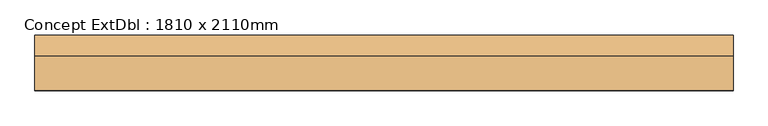
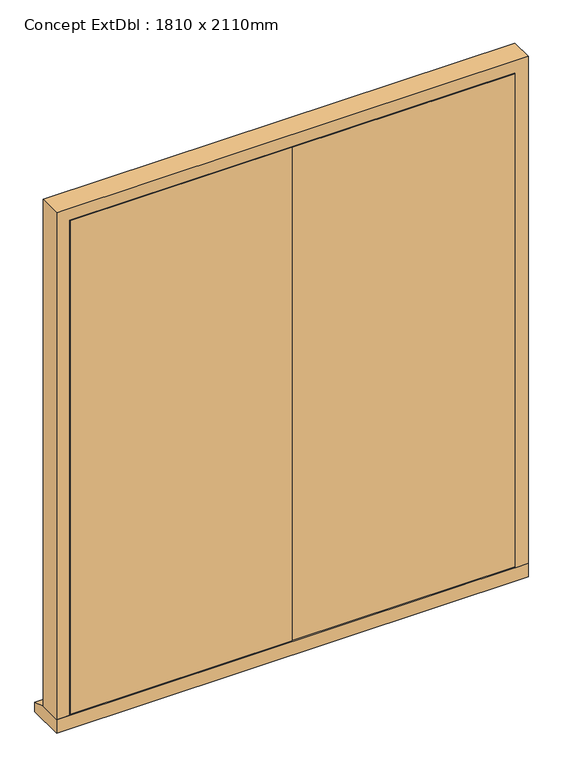
"""IFC4 building model written with IfcOpenShell, lengths in millimetres: door geometry, Concept ExtDbl : 1810 x 2110mm."""

from ifc_helpers import new_model, si_unit, frame, origin, place, context, project, spatial, polyline, outline, extrude, faceted_brep, source, transform, mapped, element, save


def concept_extdbl_1810_x_2110mm_abc10830(model_context):
    return source(origin(), model_context, "Body", "SolidModel", [
        faceted_brep([(834.5, 190.0, 54.5), (905.0, 190.0, 54.5), (905.0, 101.0, 54.5), (856.5, 101.0, 54.5), (856.5, 148.0, 54.5), (834.5, 148.0, 54.5), (834.5, 190.0, 2039.5), (-834.5, 190.0, 2039.5), (-834.5, 190.0, 54.5), (-905.0, 190.0, 54.5), (-905.0, 190.0, 2110.0), (905.0, 190.0, 2110.0), (905.0, 101.0, 2110.0), (-905.0, 101.0, 2110.0), (-905.0, 101.0, 54.5), (-856.5, 101.0, 54.5), (-856.5, 101.0, 2061.5), (856.5, 101.0, 2061.5), (856.5, 148.0, 2061.5), (-856.5, 148.0, 2061.5), (-856.5, 148.0, 54.5), (-834.5, 148.0, 54.5), (-834.5, 148.0, 2039.5), (834.5, 148.0, 2039.5)], [[[0, 1, 2, 3, 4, 5]], [[1, 0, 6, 7, 8, 9, 10, 11]], [[2, 1, 11, 12]], [[3, 2, 12, 13, 14, 15, 16, 17]], [[4, 3, 17, 18]], [[5, 4, 18, 19, 20, 21, 22, 23]], [[0, 5, 23, 6]], [[7, 22, 21, 8]], [[8, 21, 20, 15, 14, 9]], [[13, 10, 9, 14]], [[19, 16, 15, 20]], [[12, 11, 10, 13]], [[18, 17, 16, 19]], [[6, 23, 22, 7]]]),
        extrude(outline(polyline([(101.0, 0.0), (101.0, 54.5), (190.0, 54.5), (245.0, 38.5947221), (245.0, 0.0), (101.0, 0.0)])), frame((-905.0, 0.0, 0.0), z_axis=(1.0, 0.0, 0.0), x_axis=(0.0, 1.0, 0.0)), (0.0, 0.0, 1.0), 1810.0),
        extrude(outline(polyline([(853.5, 101.0), (1.5, 101.0), (1.5, 145.0), (853.5, 145.0), (853.5, 101.0)])), frame((0.0, 0.0, 58.5), z_axis=(0.0, 0.0, 1.0), x_axis=(1.0, 0.0, 0.0)), (0.0, 0.0, 1.0), 2000.0),
        extrude(outline(polyline([(-1.5, 101.0), (-853.5, 101.0), (-853.5, 145.0), (-1.5, 145.0), (-1.5, 101.0)])), frame((0.0, 0.0, 58.5), z_axis=(0.0, 0.0, 1.0), x_axis=(1.0, 0.0, 0.0)), (0.0, 0.0, 1.0), 2000.0),
    ])


if __name__ == "__main__":
    model = new_model("IFC4")
    model_context = context("Model", 3, world=origin())
    ifc_project = project(units=[si_unit("LENGTHUNIT", "METRE", prefix="MILLI")], contexts=[model_context])
    site = spatial("IfcSite", under=ifc_project)
    building = spatial("IfcBuilding", under=site)
    placement = place(None, origin())
    concept_extdbl_1810_x_2110mm_shape = concept_extdbl_1810_x_2110mm_abc10830(model_context)
    element("IfcDoor", 1, ObjectType="Concept ExtDbl : 1810 x 2110mm", at=placement, inside=building, context=model_context, shape_type="MappedRepresentation", body=[
        mapped(concept_extdbl_1810_x_2110mm_shape, transform((0.0, 0.0, 0.0), x_axis=(1.0, 0.0, 0.0), y_axis=(0.0, 1.0, 0.0), z_axis=(0.0, 0.0, 1.0))),
    ])
    save(model, "model.ifc")

# Revit data of these elements
# Type "Concept ExtDbl : 1810 x 2110mm"
#   Type Mark = "70"
#   Type Comments = "External Double"
#   Operation = "DoubleDoorSingleSwing"
#   Construction Type Id = "GSP4R"
#   Keynote = "L10"
#   Analytic Construction = "1/8 in Pilkington single glazing"
#   Visual Light Transmittance = 0.9
#   Thickness = 44 mm
#   Solar Heat Gain Coefficient = 0.78
#   Rough Width = 1810 mm
#   Rough Height = 2110 mm
#   Heat Transfer Coefficient (U) = 3.6886 W/(m²·K)
#   FrameWidth = 42 mm
#   FrameOffset - External = 25 mm
#   Height = 2110 mm
#   Width = 1810 mm
#   Define Thermal Properties by = 1
#   Function = 1
#   Material Door = Concept
#   Material Frame = Concept
#   Wall Closure = (empty or 0)
# Element 1 (IfcDoor, "Concept ExtDbl : 1810 x 2110mm")
#   Materials on its faces: "Concept"
# Materials
#   "Concept": class "Miscellaneous", colour RGB 128 128 255, transparency 0.5
